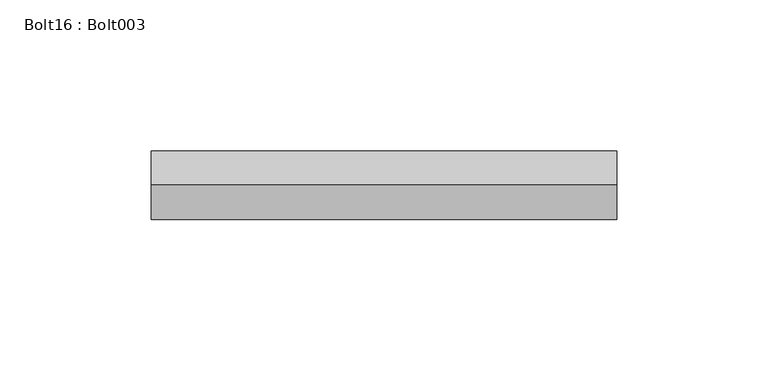
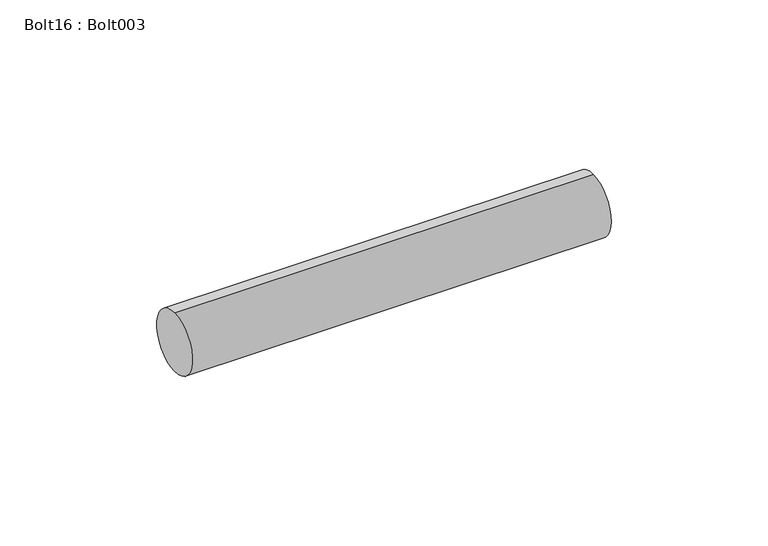
"""IFC4 building model written with IfcOpenShell, lengths in millimetres: proxy geometry, Bolt16 : Bolt003."""

import ifcopenshell
import ifcopenshell.guid

model = None  # the IFC model being written
_history = None  # IfcOwnerHistory: only IFC2X3 demands one
_inside = {}  # id of a spatial element -> (the spatial element, [elements in it])
_under = {}  # id of a project, library or spatial element -> (it, [spatial elements below it])
_declared = {}  # id of a project -> (the project, [libraries it declares])
_typed = {}  # id of a type object -> (the type object, [elements of that type])
_made_of = {}  # id of a material, layer set ... -> (it, [elements and type objects made of it])


def new_model(schema):
    """Start an empty IFC model of exactly this schema.

    Asked for "IFC4X3", IfcOpenShell would pick the latest addendum, in which some entities
    have other attributes; the version numbers below select the first issue.
    IFC2X3 requires an IfcOwnerHistory on every rooted entity: one is made here for all.
    """
    global model, _history
    if schema == "IFC4X3":
        model = ifcopenshell.file(schema_version=(4, 3, 0, 0))
    else:
        model = ifcopenshell.file(schema=schema)
    _inside.clear()
    _under.clear()
    _declared.clear()
    _typed.clear()
    _made_of.clear()
    _history = None
    if model.schema == "IFC2X3":
        org = make("IfcOrganization", Name="unknown")
        user = make(
            "IfcPersonAndOrganization",
            ThePerson=make("IfcPerson", FamilyName="unknown"),
            TheOrganization=org,
        )
        app = make(
            "IfcApplication",
            ApplicationDeveloper=org,
            Version="unknown",
            ApplicationFullName="unknown",
            ApplicationIdentifier="unknown",
        )
        _history = make(
            "IfcOwnerHistory",
            OwningUser=user,
            OwningApplication=app,
            ChangeAction="ADDED",
            CreationDate=0,
        )
    return model


def make(cls, **values):
    """One entity of the class cls with the attributes given. An attribute that is None is left unset."""
    return model.create_entity(
        cls, **{name: value for name, value in values.items() if value is not None}
    )


def rooted(cls, **values):
    """An entity with a GlobalId (a new one), such as an element, a storey or a relation."""
    return make(cls, GlobalId=ifcopenshell.guid.new(), OwnerHistory=_history, **values)


def si_unit(unit_type, name, prefix=None):
    """IfcSIUnit, for example si_unit("LENGTHUNIT", "METRE", prefix="MILLI")."""
    return make("IfcSIUnit", UnitType=unit_type, Prefix=prefix, Name=name)


def assignment(units):
    """IfcUnitAssignment: the units of a project."""
    return None if units is None else make("IfcUnitAssignment", Units=units)


def point(xyz):
    """IfcCartesianPoint."""
    return None if xyz is None else make("IfcCartesianPoint", Coordinates=xyz)


def direction(xyz):
    """IfcDirection."""
    return None if xyz is None else make("IfcDirection", DirectionRatios=xyz)


def frame(location, z_axis=None, x_axis=None):
    """IfcAxis2Placement3D, a coordinate frame: its origin and axes. An axis left out is left unset."""
    return make(
        "IfcAxis2Placement3D",
        Location=point(location),
        Axis=direction(z_axis),
        RefDirection=direction(x_axis),
    )


def frame_2d(location, x_axis=None):
    """IfcAxis2Placement2D, a coordinate frame in the plane: its origin and x axis."""
    return make(
        "IfcAxis2Placement2D", Location=point(location), RefDirection=direction(x_axis)
    )


def origin():
    """The frame at (0, 0, 0) with its axes left unset."""
    return frame((0.0, 0.0, 0.0))


def place(relative_to, where):
    """IfcLocalPlacement: puts the frame where relative to a parent placement (None: the world)."""
    return make(
        "IfcLocalPlacement", PlacementRelTo=relative_to, RelativePlacement=where
    )


def context(
    kind, dimensions, precision=None, world=None, true_north=None, identifier=None
):
    """IfcGeometricRepresentationContext, for example the 3D "Model" context."""
    return make(
        "IfcGeometricRepresentationContext",
        ContextIdentifier=identifier,
        ContextType=kind,
        CoordinateSpaceDimension=dimensions,
        Precision=precision,
        WorldCoordinateSystem=world,
        TrueNorth=true_north,
    )


def project(units=None, contexts=None):
    """IfcProject with its units and contexts."""
    return rooted(
        "IfcProject",
        Name="project",
        RepresentationContexts=contexts,
        UnitsInContext=assignment(units),
    )


def spatial(cls, under=None, at=None, **own):
    """A site, building, storey or space (cls), placed at a placement, below another one or the project."""
    s = rooted(cls, ObjectPlacement=at, **own)
    if under is not None:
        _under.setdefault(under.id(), (under, []))[1].append(s)
    return s


def circle_curve(where, radius):
    """IfcCircle in the frame where."""
    return make("IfcCircle", Position=where, Radius=radius)


def trimmed(basis, trim1, trim2, sense, master):
    """IfcTrimmedCurve: the piece of a basis curve between two trims."""
    return make(
        "IfcTrimmedCurve",
        BasisCurve=basis,
        Trim1=trim1,
        Trim2=trim2,
        SenseAgreement=sense,
        MasterRepresentation=master,
    )


def segment(curve, same_sense, transition):
    """IfcCompositeCurveSegment."""
    return make(
        "IfcCompositeCurveSegment",
        Transition=transition,
        SameSense=same_sense,
        ParentCurve=curve,
    )


def composite_curve(segments, self_intersect=None):
    """IfcCompositeCurve: segments joined end to end."""
    return make("IfcCompositeCurve", Segments=segments, SelfIntersect=self_intersect)


def outline(outer, holes=None, kind="AREA"):
    """IfcArbitraryClosedProfileDef: a profile drawn as a closed curve; with holes, ...WithVoids."""
    if holes is None:
        return make("IfcArbitraryClosedProfileDef", ProfileType=kind, OuterCurve=outer)
    return make(
        "IfcArbitraryProfileDefWithVoids",
        ProfileType=kind,
        OuterCurve=outer,
        InnerCurves=holes,
    )


def extrude(swept, where, along, depth):
    """IfcExtrudedAreaSolid: the profile swept, set in the frame where, extruded along a direction by depth."""
    return make(
        "IfcExtrudedAreaSolid",
        SweptArea=swept,
        Position=where,
        ExtrudedDirection=direction(along),
        Depth=depth,
    )


def shape(context_of_items, identifier, shape_type, items):
    """IfcShapeRepresentation: the items that make up one representation, for example the "Body"."""
    return make(
        "IfcShapeRepresentation",
        ContextOfItems=context_of_items,
        RepresentationIdentifier=identifier,
        RepresentationType=shape_type,
        Items=items,
    )


def source(mapping_origin, context_of_items, identifier, shape_type, items):
    """IfcRepresentationMap: a shape defined once, which mapped items show again and again."""
    return make(
        "IfcRepresentationMap",
        MappingOrigin=mapping_origin,
        MappedRepresentation=shape(context_of_items, identifier, shape_type, items),
    )


def transform(
    local_origin,
    x_axis=None,
    y_axis=None,
    z_axis=None,
    scale=None,
    scale2=None,
    scale3=None,
    uniform=True,
):
    """IfcCartesianTransformationOperator3D, or its non-uniform kind. x_axis, y_axis, z_axis: its Axis1, 2, 3."""
    if uniform:
        return make(
            "IfcCartesianTransformationOperator3D",
            Axis1=direction(x_axis),
            Axis2=direction(y_axis),
            LocalOrigin=point(local_origin),
            Scale=scale,
            Axis3=direction(z_axis),
        )
    return make(
        "IfcCartesianTransformationOperator3DnonUniform",
        Axis1=direction(x_axis),
        Axis2=direction(y_axis),
        LocalOrigin=point(local_origin),
        Scale=scale,
        Axis3=direction(z_axis),
        Scale2=scale2,
        Scale3=scale3,
    )


def mapped(mapping_source, mapping_target):
    """IfcMappedItem: shows the shape of a source again, moved by a transform."""
    return make(
        "IfcMappedItem", MappingSource=mapping_source, MappingTarget=mapping_target
    )


def made_of(thing, what):
    """Note that an element or type object is made of a material, layer set ...; save() writes the relation."""
    if what is not None:
        _made_of.setdefault(what.id(), (what, []))[1].append(thing)
    return thing


def element(
    cls,
    number,
    at=None,
    inside=None,
    cuts=None,
    type_object=None,
    material=None,
    context=None,
    identifier="Body",
    shape_type=None,
    held_by="IfcProductDefinitionShape",
    body=None,
    shapes=None,
    **own,
):
    """One element of the class cls, such as IfcWall. Its Tag is "e" and its number.

    at: its placement. inside: the storey or other place that contains it. cuts: it is an
    opening in that element (IfcRelVoidsElement). A single representation is given by context,
    identifier, shape_type and body (its items); several are given by shapes. held_by: the class
    of the entity that holds the representations. save() writes the other relations.
    """
    e = rooted(cls, Tag="e%d" % number, ObjectPlacement=at, **own)
    if body is not None:
        shapes = [shape(context, identifier, shape_type, body)]
    if shapes is not None:
        e.Representation = make(held_by, Representations=shapes)
    if inside is not None:
        _inside.setdefault(inside.id(), (inside, []))[1].append(e)
    if cuts is not None:
        rooted(
            "IfcRelVoidsElement", RelatingBuildingElement=cuts, RelatedOpeningElement=e
        )
    if type_object is not None:
        _typed.setdefault(type_object.id(), (type_object, []))[1].append(e)
    return made_of(e, material)


def aggregate(whole, parts):
    """IfcRelAggregates: a whole, such as a stair, and the parts it consists of."""
    return rooted("IfcRelAggregates", RelatingObject=whole, RelatedObjects=parts)


def save(model, path):
    """Write the relations noted so far, then the file.

    IfcRelAggregates (storeys below a building ...), IfcRelContainedInSpatialStructure (elements
    in a storey), IfcRelDefinesByType, IfcRelAssociatesMaterial and IfcRelDeclares: one each for
    every whole, place, type object, material and project.
    """
    for whole, parts in _under.values():
        aggregate(whole, parts)
    for where, things in _inside.values():
        rooted(
            "IfcRelContainedInSpatialStructure",
            RelatedElements=things,
            RelatingStructure=where,
        )
    for kind, things in _typed.values():
        rooted("IfcRelDefinesByType", RelatedObjects=things, RelatingType=kind)
    for what, things in _made_of.values():
        rooted("IfcRelAssociatesMaterial", RelatedObjects=things, RelatingMaterial=what)
    for by, libraries in _declared.values():
        rooted("IfcRelDeclares", RelatingContext=by, RelatedDefinitions=libraries)
    model.write(path)


def bolt16_bolt003_f80aea55(model_context):
    return source(origin(), model_context, "Body", "SweptSolid", [
        extrude(outline(composite_curve([segment(trimmed(circle_curve(frame_2d((1896.5882072, 39910.0063132)), 11.4045168), [point((1896.5882072, 39921.41083))], [point((1896.5882072, 39898.6017964))], False, "CARTESIAN"), True, "CONTINUOUS"), segment(trimmed(circle_curve(frame_2d((1896.5882072, 39910.0063132)), 11.4045168), [point((1896.5882072, 39898.6017964))], [point((1896.5882072, 39921.41083))], False, "CARTESIAN"), True, "CONTINUOUS")], self_intersect=False)), frame((10287.3140827, 0.0, 0.0), z_axis=(1.0, 0.0, 0.0), x_axis=(0.0, 1.0, 0.0)), (0.0, 0.0, 1.0), 154.0602393),
    ])


if __name__ == "__main__":
    model = new_model("IFC4")
    model_context = context("Model", 3, world=origin())
    ifc_project = project(units=[si_unit("LENGTHUNIT", "METRE", prefix="MILLI")], contexts=[model_context])
    site = spatial("IfcSite", under=ifc_project)
    building = spatial("IfcBuilding", under=site)
    placement = place(None, origin())
    bolt16_bolt003_shape = bolt16_bolt003_f80aea55(model_context)
    element("IfcBuildingElementProxy", 1, Name="Bolt16 : Bolt003", ObjectType="Bolt16 : Bolt003", at=placement, inside=building, context=model_context, shape_type="MappedRepresentation", body=[
        mapped(bolt16_bolt003_shape, transform((0.0, 0.0, 0.0), x_axis=(1.0, 0.0, 0.0), y_axis=(0.0, 1.0, 0.0), z_axis=(0.0, 0.0, 1.0))),
    ])
    save(model, "model.ifc")

# Revit data of these elements
# Type "Bolt16 : Bolt003"
#   NameOverride = "Bolt003"
# Element 1 (IfcBuildingElementProxy, "Bolt16 : Bolt003")
#   Materials on its faces: "TUBE STEEL STRINGER WELDED TO ANCHORED STEEL PLATE - SEE STRUCT DWGS"
# Materials
#   "TUBE STEEL STRINGER WELDED TO ANCHORED STEEL PLATE - SEE STRUCT DWGS": class "Unassigned", colour RGB 128 128 128, transparency 0, Cost = 0
